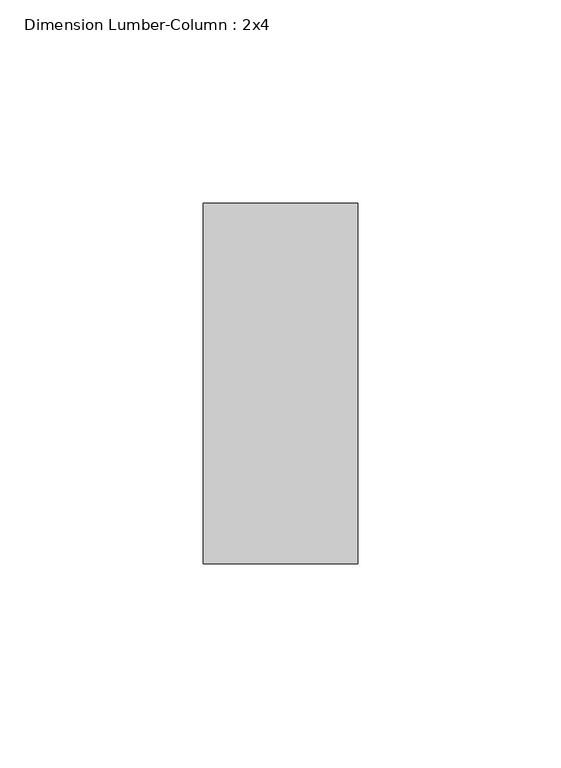
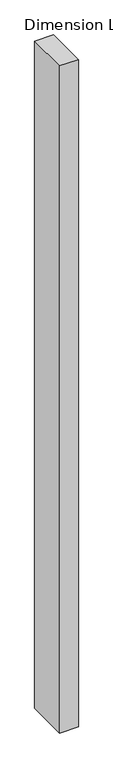
"""IFC4 building model written with IfcOpenShell, lengths in millimetres: column geometry, Dimension Lumber-Column : 2x4."""

from ifc_helpers import new_model, si_unit, frame, origin, place, context, project, spatial, polyline, outline, extrude, source, transform, mapped, element, save


def dimension_lumber_column_2x4_c4e013fe(model_context):
    return source(origin(), model_context, "Body", "SweptSolid", [
        extrude(outline(polyline([(19.05, 44.45), (19.05, -44.45), (-19.05, -44.45), (-19.05, 44.45), (19.05, 44.45)])), frame((0.0, 0.0, 56.35625), z_axis=(0.0, 0.0, 1.0), x_axis=(1.0, 0.0, 0.0)), (0.0, 0.0, 1.0), 1444.228125),
    ])


if __name__ == "__main__":
    model = new_model("IFC4")
    model_context = context("Model", 3, world=origin())
    ifc_project = project(units=[si_unit("LENGTHUNIT", "METRE", prefix="MILLI")], contexts=[model_context])
    site = spatial("IfcSite", under=ifc_project)
    building = spatial("IfcBuilding", under=site)
    placement = place(None, origin())
    dimension_lumber_column_2x4_shape = dimension_lumber_column_2x4_c4e013fe(model_context)
    element("IfcColumn", 1, ObjectType="Dimension Lumber-Column : 2x4", at=placement, inside=building, context=model_context, shape_type="MappedRepresentation", body=[
        mapped(dimension_lumber_column_2x4_shape, transform((0.0, 0.0, 0.0), x_axis=(1.0, 0.0, 0.0), y_axis=(0.0, 1.0, 0.0), z_axis=(0.0, 0.0, 1.0))),
    ])
    save(model, "model.ifc")

# Revit data of these elements
# Type "Dimension Lumber-Column : 2x4"
#   Int Type = "Interior"
#   Assembly Code = "B10"
#   Cost = 8.05
#   A = 0.0364583 SF
#   b = 0' - 1 1/2"
#   d = 0' - 3 1/2"
#   Structural Material [instance default] = Softwood, Lumber
# Element 1 (IfcColumn, "Dimension Lumber-Column : 2x4")
#   Structural Material = Douglas Fir #2
#   Materials on its faces: "Douglas Fir #2"
# Materials
#   "Softwood, Lumber": class "Wood", colour RGB 223 192 134, transparency 0, Description = "Pinus Echinata", Cost = 0
#   "Douglas Fir #2": class "Wood", colour RGB 223 192 134, transparency 0, Description = "Pinus Echinata", Cost = 0
